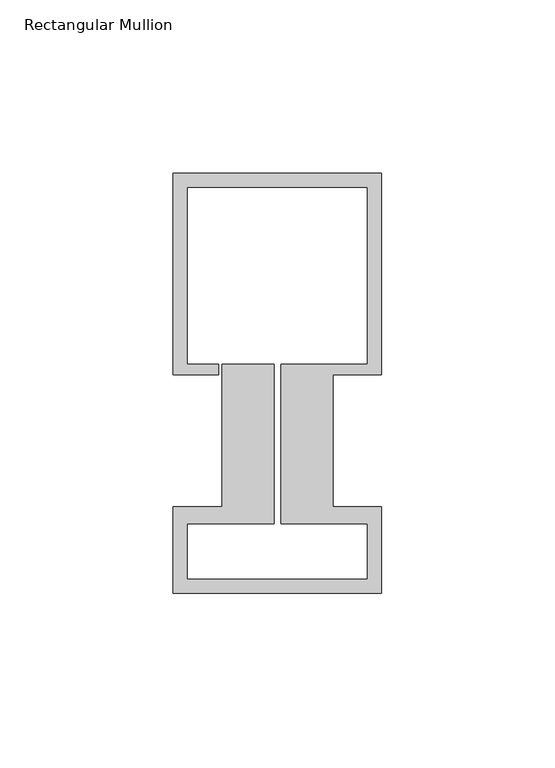
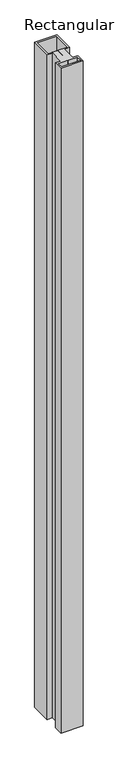
"""IFC4 building model written with IfcOpenShell, lengths in millimetres: member geometry, Rectangular Mullion : Schueco_FWS-60-SI_Tran_CovCap-20mm_Tran-55mm."""

from ifc_helpers import new_model, si_unit, frame, origin, place, context, project, spatial, polyline, outline, extrude, source, transform, mapped, element, save


def rectangular_mullion_1ff48283(model_context):
    return source(origin(), model_context, "Body", "SweptSolid", [
        extrude(outline(polyline([(0.0, 96.0), (0.0, 38.0), (-14.0, 38.0), (-14.0, -0.1), (0.0, -0.1), (0.0, -25.0), (-60.0, -25.0), (-60.0, -0.1), (-46.0, -0.1), (-46.0, 41.0), (-31.0, 41.0), (-31.0, -5.0), (-56.0, -5.0), (-56.0, -21.0), (-4.0, -21.0), (-4.0, -5.0), (-29.0, -5.0), (-29.0, 41.0), (-4.0, 41.0), (-4.0, 92.0), (-56.0, 92.0), (-56.0, 41.0), (-47.0, 41.0), (-47.0, 38.0), (-60.0, 38.0), (-60.0, 96.0), (0.0, 96.0)])), frame((0.0, 0.0, -1880.0), z_axis=(0.0, 0.0, 1.0), x_axis=(1.0, 0.0, 0.0)), (0.0, 0.0, 1.0), 1880.0),
    ])


if __name__ == "__main__":
    model = new_model("IFC4")
    model_context = context("Model", 3, world=origin())
    ifc_project = project(units=[si_unit("LENGTHUNIT", "METRE", prefix="MILLI")], contexts=[model_context])
    site = spatial("IfcSite", under=ifc_project)
    building = spatial("IfcBuilding", under=site)
    placement = place(None, origin())
    rectangular_mullion_shape = rectangular_mullion_1ff48283(model_context)
    element("IfcMember", 1, ObjectType="Rectangular Mullion : Schueco_FWS-60-SI_Tran_CovCap-20mm_Tran-55mm", at=placement, inside=building, context=model_context, shape_type="MappedRepresentation", body=[
        mapped(rectangular_mullion_shape, transform((0.0, 0.0, 0.0), x_axis=(1.0, 0.0, 0.0), y_axis=(0.0, 1.0, 0.0), z_axis=(0.0, 0.0, 1.0))),
    ])
    save(model, "model.ifc")

# Revit data of these elements
# Type "Rectangular Mullion : Schueco_FWS-60-SI_Tran_CovCap-20mm_Tran-55mm"
#   Model = "FWS 60.SI"
#   Manufacturer = "Schueco International KG"
#   Type Comments = "Transom"
#   Schueco thermal insulation standard = "Suitable for passive houses"
#   Burglar resistance = "RC 3"
#   Thermal insulation = "to 0.70 W/(m²K)"
#   built-in parameter 1007322 = 0.396982 (stored number, unit not read)
#   built-in parameter 1007321 = 0.0524934 (stored number, unit not read)
#   built-in parameter 1007320 = 0.0524934 (stored number, unit not read)
# Element 1 (IfcMember, "Rectangular Mullion : Schueco_FWS-60-SI_Tran_CovCap-20mm_Tran-55mm")
#   Materials on its faces: "Alu"
# Materials
#   "Alu": class "Glas", colour RGB 140 140 140, transparency 0
